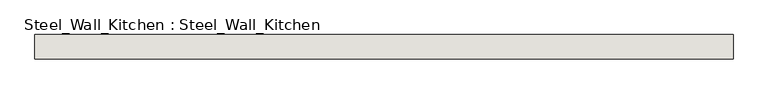
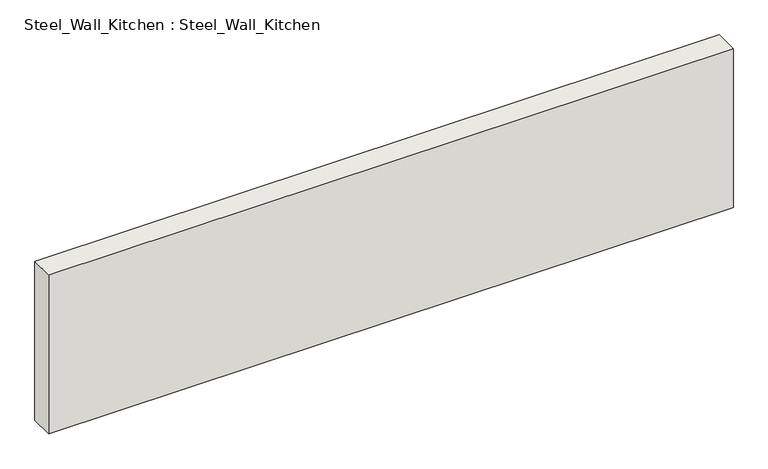
"""IFC4 building model written with IfcOpenShell, lengths in millimetres: wall geometry, Steel_Wall_Kitchen : Steel_Wall_Kitchen."""

import ifcopenshell
import ifcopenshell.guid

model = None  # the IFC model being written
_history = None  # IfcOwnerHistory: only IFC2X3 demands one
_inside = {}  # id of a spatial element -> (the spatial element, [elements in it])
_under = {}  # id of a project, library or spatial element -> (it, [spatial elements below it])
_declared = {}  # id of a project -> (the project, [libraries it declares])
_typed = {}  # id of a type object -> (the type object, [elements of that type])
_made_of = {}  # id of a material, layer set ... -> (it, [elements and type objects made of it])


def new_model(schema):
    """Start an empty IFC model of exactly this schema.

    Asked for "IFC4X3", IfcOpenShell would pick the latest addendum, in which some entities
    have other attributes; the version numbers below select the first issue.
    IFC2X3 requires an IfcOwnerHistory on every rooted entity: one is made here for all.
    """
    global model, _history
    if schema == "IFC4X3":
        model = ifcopenshell.file(schema_version=(4, 3, 0, 0))
    else:
        model = ifcopenshell.file(schema=schema)
    _inside.clear()
    _under.clear()
    _declared.clear()
    _typed.clear()
    _made_of.clear()
    _history = None
    if model.schema == "IFC2X3":
        org = make("IfcOrganization", Name="unknown")
        user = make(
            "IfcPersonAndOrganization",
            ThePerson=make("IfcPerson", FamilyName="unknown"),
            TheOrganization=org,
        )
        app = make(
            "IfcApplication",
            ApplicationDeveloper=org,
            Version="unknown",
            ApplicationFullName="unknown",
            ApplicationIdentifier="unknown",
        )
        _history = make(
            "IfcOwnerHistory",
            OwningUser=user,
            OwningApplication=app,
            ChangeAction="ADDED",
            CreationDate=0,
        )
    return model


def make(cls, **values):
    """One entity of the class cls with the attributes given. An attribute that is None is left unset."""
    return model.create_entity(
        cls, **{name: value for name, value in values.items() if value is not None}
    )


def rooted(cls, **values):
    """An entity with a GlobalId (a new one), such as an element, a storey or a relation."""
    return make(cls, GlobalId=ifcopenshell.guid.new(), OwnerHistory=_history, **values)


def si_unit(unit_type, name, prefix=None):
    """IfcSIUnit, for example si_unit("LENGTHUNIT", "METRE", prefix="MILLI")."""
    return make("IfcSIUnit", UnitType=unit_type, Prefix=prefix, Name=name)


def assignment(units):
    """IfcUnitAssignment: the units of a project."""
    return None if units is None else make("IfcUnitAssignment", Units=units)


def point(xyz):
    """IfcCartesianPoint."""
    return None if xyz is None else make("IfcCartesianPoint", Coordinates=xyz)


def direction(xyz):
    """IfcDirection."""
    return None if xyz is None else make("IfcDirection", DirectionRatios=xyz)


def frame(location, z_axis=None, x_axis=None):
    """IfcAxis2Placement3D, a coordinate frame: its origin and axes. An axis left out is left unset."""
    return make(
        "IfcAxis2Placement3D",
        Location=point(location),
        Axis=direction(z_axis),
        RefDirection=direction(x_axis),
    )


def origin():
    """The frame at (0, 0, 0) with its axes left unset."""
    return frame((0.0, 0.0, 0.0))


def place(relative_to, where):
    """IfcLocalPlacement: puts the frame where relative to a parent placement (None: the world)."""
    return make(
        "IfcLocalPlacement", PlacementRelTo=relative_to, RelativePlacement=where
    )


def context(
    kind, dimensions, precision=None, world=None, true_north=None, identifier=None
):
    """IfcGeometricRepresentationContext, for example the 3D "Model" context."""
    return make(
        "IfcGeometricRepresentationContext",
        ContextIdentifier=identifier,
        ContextType=kind,
        CoordinateSpaceDimension=dimensions,
        Precision=precision,
        WorldCoordinateSystem=world,
        TrueNorth=true_north,
    )


def project(units=None, contexts=None):
    """IfcProject with its units and contexts."""
    return rooted(
        "IfcProject",
        Name="project",
        RepresentationContexts=contexts,
        UnitsInContext=assignment(units),
    )


def spatial(cls, under=None, at=None, **own):
    """A site, building, storey or space (cls), placed at a placement, below another one or the project."""
    s = rooted(cls, ObjectPlacement=at, **own)
    if under is not None:
        _under.setdefault(under.id(), (under, []))[1].append(s)
    return s


def polyline(points):
    """IfcPolyline through the points."""
    return make("IfcPolyline", Points=[point(p) for p in points])


def outline(outer, holes=None, kind="AREA"):
    """IfcArbitraryClosedProfileDef: a profile drawn as a closed curve; with holes, ...WithVoids."""
    if holes is None:
        return make("IfcArbitraryClosedProfileDef", ProfileType=kind, OuterCurve=outer)
    return make(
        "IfcArbitraryProfileDefWithVoids",
        ProfileType=kind,
        OuterCurve=outer,
        InnerCurves=holes,
    )


def extrude(swept, where, along, depth):
    """IfcExtrudedAreaSolid: the profile swept, set in the frame where, extruded along a direction by depth."""
    return make(
        "IfcExtrudedAreaSolid",
        SweptArea=swept,
        Position=where,
        ExtrudedDirection=direction(along),
        Depth=depth,
    )


def shape(context_of_items, identifier, shape_type, items):
    """IfcShapeRepresentation: the items that make up one representation, for example the "Body"."""
    return make(
        "IfcShapeRepresentation",
        ContextOfItems=context_of_items,
        RepresentationIdentifier=identifier,
        RepresentationType=shape_type,
        Items=items,
    )


def source(mapping_origin, context_of_items, identifier, shape_type, items):
    """IfcRepresentationMap: a shape defined once, which mapped items show again and again."""
    return make(
        "IfcRepresentationMap",
        MappingOrigin=mapping_origin,
        MappedRepresentation=shape(context_of_items, identifier, shape_type, items),
    )


def transform(
    local_origin,
    x_axis=None,
    y_axis=None,
    z_axis=None,
    scale=None,
    scale2=None,
    scale3=None,
    uniform=True,
):
    """IfcCartesianTransformationOperator3D, or its non-uniform kind. x_axis, y_axis, z_axis: its Axis1, 2, 3."""
    if uniform:
        return make(
            "IfcCartesianTransformationOperator3D",
            Axis1=direction(x_axis),
            Axis2=direction(y_axis),
            LocalOrigin=point(local_origin),
            Scale=scale,
            Axis3=direction(z_axis),
        )
    return make(
        "IfcCartesianTransformationOperator3DnonUniform",
        Axis1=direction(x_axis),
        Axis2=direction(y_axis),
        LocalOrigin=point(local_origin),
        Scale=scale,
        Axis3=direction(z_axis),
        Scale2=scale2,
        Scale3=scale3,
    )


def mapped(mapping_source, mapping_target):
    """IfcMappedItem: shows the shape of a source again, moved by a transform."""
    return make(
        "IfcMappedItem", MappingSource=mapping_source, MappingTarget=mapping_target
    )


def made_of(thing, what):
    """Note that an element or type object is made of a material, layer set ...; save() writes the relation."""
    if what is not None:
        _made_of.setdefault(what.id(), (what, []))[1].append(thing)
    return thing


def element(
    cls,
    number,
    at=None,
    inside=None,
    cuts=None,
    type_object=None,
    material=None,
    context=None,
    identifier="Body",
    shape_type=None,
    held_by="IfcProductDefinitionShape",
    body=None,
    shapes=None,
    **own,
):
    """One element of the class cls, such as IfcWall. Its Tag is "e" and its number.

    at: its placement. inside: the storey or other place that contains it. cuts: it is an
    opening in that element (IfcRelVoidsElement). A single representation is given by context,
    identifier, shape_type and body (its items); several are given by shapes. held_by: the class
    of the entity that holds the representations. save() writes the other relations.
    """
    e = rooted(cls, Tag="e%d" % number, ObjectPlacement=at, **own)
    if body is not None:
        shapes = [shape(context, identifier, shape_type, body)]
    if shapes is not None:
        e.Representation = make(held_by, Representations=shapes)
    if inside is not None:
        _inside.setdefault(inside.id(), (inside, []))[1].append(e)
    if cuts is not None:
        rooted(
            "IfcRelVoidsElement", RelatingBuildingElement=cuts, RelatedOpeningElement=e
        )
    if type_object is not None:
        _typed.setdefault(type_object.id(), (type_object, []))[1].append(e)
    return made_of(e, material)


def aggregate(whole, parts):
    """IfcRelAggregates: a whole, such as a stair, and the parts it consists of."""
    return rooted("IfcRelAggregates", RelatingObject=whole, RelatedObjects=parts)


def save(model, path):
    """Write the relations noted so far, then the file.

    IfcRelAggregates (storeys below a building ...), IfcRelContainedInSpatialStructure (elements
    in a storey), IfcRelDefinesByType, IfcRelAssociatesMaterial and IfcRelDeclares: one each for
    every whole, place, type object, material and project.
    """
    for whole, parts in _under.values():
        aggregate(whole, parts)
    for where, things in _inside.values():
        rooted(
            "IfcRelContainedInSpatialStructure",
            RelatedElements=things,
            RelatingStructure=where,
        )
    for kind, things in _typed.values():
        rooted("IfcRelDefinesByType", RelatedObjects=things, RelatingType=kind)
    for what, things in _made_of.values():
        rooted("IfcRelAssociatesMaterial", RelatedObjects=things, RelatingMaterial=what)
    for by, libraries in _declared.values():
        rooted("IfcRelDeclares", RelatingContext=by, RelatedDefinitions=libraries)
    model.write(path)


def steel_wall_kitchen_steel_wall_kitchen_7f8e7296(model_context):
    return source(origin(), model_context, "Body", "SweptSolid", [
        extrude(outline(polyline([(4365.0, 9495.0), (1515.0, 9495.0), (1515.0, 9595.0), (4365.0, 9595.0), (4365.0, 9495.0)])), frame((0.0, 0.0, 2850.0), z_axis=(0.0, 0.0, 1.0), x_axis=(1.0, 0.0, 0.0)), (0.0, 0.0, 1.0), 700.0),
    ])


if __name__ == "__main__":
    model = new_model("IFC4")
    model_context = context("Model", 3, world=origin())
    ifc_project = project(units=[si_unit("LENGTHUNIT", "METRE", prefix="MILLI")], contexts=[model_context])
    site = spatial("IfcSite", under=ifc_project)
    building = spatial("IfcBuilding", under=site)
    placement = place(None, origin())
    steel_wall_kitchen_steel_wall_kitchen_shape = steel_wall_kitchen_steel_wall_kitchen_7f8e7296(model_context)
    element("IfcWall", 1, ObjectType="Steel_Wall_Kitchen : Steel_Wall_Kitchen", at=placement, inside=building, context=model_context, shape_type="MappedRepresentation", body=[
        mapped(steel_wall_kitchen_steel_wall_kitchen_shape, transform((0.0, 0.0, 0.0), x_axis=(1.0, 0.0, 0.0), y_axis=(0.0, 1.0, 0.0), z_axis=(0.0, 0.0, 1.0))),
    ])
    save(model, "model.ifc")

# Revit data of these elements
# Type "Steel_Wall_Kitchen : Steel_Wall_Kitchen"
#   NameOverride = "Steel_Wall_Kitchen"
# Element 1 (IfcWall, "Steel_Wall_Kitchen : Steel_Wall_Kitchen")
#   Materials on its faces: "IfcSurfaceStyle #33"
# Materials
#   "IfcSurfaceStyle #33": class "Unassigned", colour RGB 214 214 214, transparency 0
